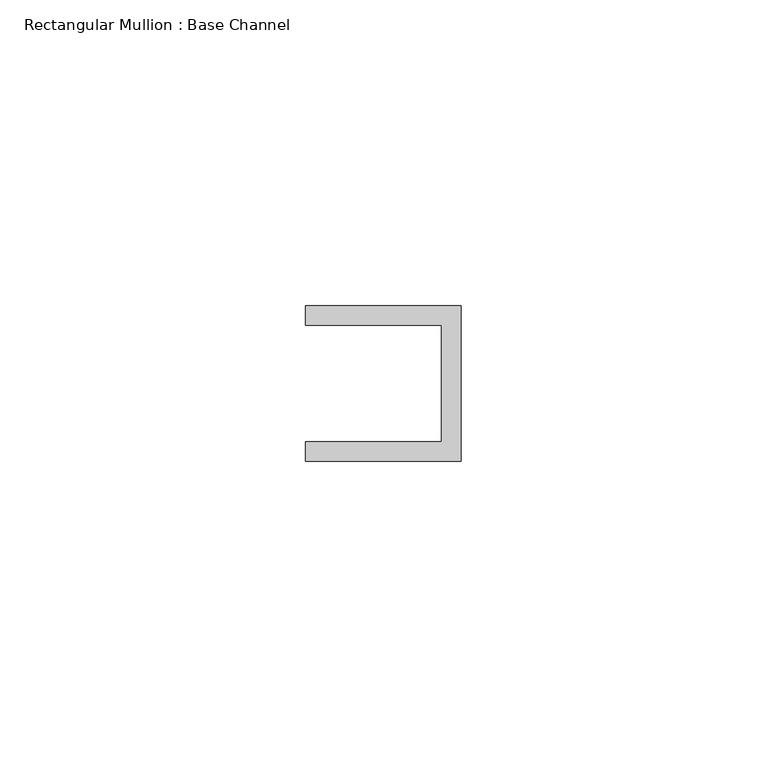
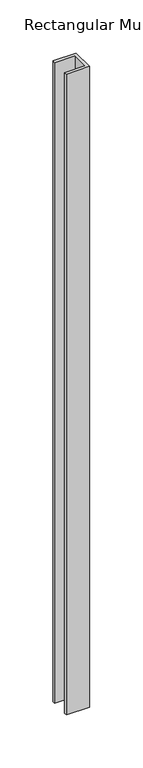
"""IFC4 building model written with IfcOpenShell, lengths in millimetres: member geometry, Rectangular Mullion : Base Channel."""

import ifcopenshell
import ifcopenshell.guid

model = None  # the IFC model being written
_history = None  # IfcOwnerHistory: only IFC2X3 demands one
_inside = {}  # id of a spatial element -> (the spatial element, [elements in it])
_under = {}  # id of a project, library or spatial element -> (it, [spatial elements below it])
_declared = {}  # id of a project -> (the project, [libraries it declares])
_typed = {}  # id of a type object -> (the type object, [elements of that type])
_made_of = {}  # id of a material, layer set ... -> (it, [elements and type objects made of it])


def new_model(schema):
    """Start an empty IFC model of exactly this schema.

    Asked for "IFC4X3", IfcOpenShell would pick the latest addendum, in which some entities
    have other attributes; the version numbers below select the first issue.
    IFC2X3 requires an IfcOwnerHistory on every rooted entity: one is made here for all.
    """
    global model, _history
    if schema == "IFC4X3":
        model = ifcopenshell.file(schema_version=(4, 3, 0, 0))
    else:
        model = ifcopenshell.file(schema=schema)
    _inside.clear()
    _under.clear()
    _declared.clear()
    _typed.clear()
    _made_of.clear()
    _history = None
    if model.schema == "IFC2X3":
        org = make("IfcOrganization", Name="unknown")
        user = make(
            "IfcPersonAndOrganization",
            ThePerson=make("IfcPerson", FamilyName="unknown"),
            TheOrganization=org,
        )
        app = make(
            "IfcApplication",
            ApplicationDeveloper=org,
            Version="unknown",
            ApplicationFullName="unknown",
            ApplicationIdentifier="unknown",
        )
        _history = make(
            "IfcOwnerHistory",
            OwningUser=user,
            OwningApplication=app,
            ChangeAction="ADDED",
            CreationDate=0,
        )
    return model


def make(cls, **values):
    """One entity of the class cls with the attributes given. An attribute that is None is left unset."""
    return model.create_entity(
        cls, **{name: value for name, value in values.items() if value is not None}
    )


def rooted(cls, **values):
    """An entity with a GlobalId (a new one), such as an element, a storey or a relation."""
    return make(cls, GlobalId=ifcopenshell.guid.new(), OwnerHistory=_history, **values)


def si_unit(unit_type, name, prefix=None):
    """IfcSIUnit, for example si_unit("LENGTHUNIT", "METRE", prefix="MILLI")."""
    return make("IfcSIUnit", UnitType=unit_type, Prefix=prefix, Name=name)


def assignment(units):
    """IfcUnitAssignment: the units of a project."""
    return None if units is None else make("IfcUnitAssignment", Units=units)


def point(xyz):
    """IfcCartesianPoint."""
    return None if xyz is None else make("IfcCartesianPoint", Coordinates=xyz)


def direction(xyz):
    """IfcDirection."""
    return None if xyz is None else make("IfcDirection", DirectionRatios=xyz)


def frame(location, z_axis=None, x_axis=None):
    """IfcAxis2Placement3D, a coordinate frame: its origin and axes. An axis left out is left unset."""
    return make(
        "IfcAxis2Placement3D",
        Location=point(location),
        Axis=direction(z_axis),
        RefDirection=direction(x_axis),
    )


def origin():
    """The frame at (0, 0, 0) with its axes left unset."""
    return frame((0.0, 0.0, 0.0))


def place(relative_to, where):
    """IfcLocalPlacement: puts the frame where relative to a parent placement (None: the world)."""
    return make(
        "IfcLocalPlacement", PlacementRelTo=relative_to, RelativePlacement=where
    )


def context(
    kind, dimensions, precision=None, world=None, true_north=None, identifier=None
):
    """IfcGeometricRepresentationContext, for example the 3D "Model" context."""
    return make(
        "IfcGeometricRepresentationContext",
        ContextIdentifier=identifier,
        ContextType=kind,
        CoordinateSpaceDimension=dimensions,
        Precision=precision,
        WorldCoordinateSystem=world,
        TrueNorth=true_north,
    )


def project(units=None, contexts=None):
    """IfcProject with its units and contexts."""
    return rooted(
        "IfcProject",
        Name="project",
        RepresentationContexts=contexts,
        UnitsInContext=assignment(units),
    )


def spatial(cls, under=None, at=None, **own):
    """A site, building, storey or space (cls), placed at a placement, below another one or the project."""
    s = rooted(cls, ObjectPlacement=at, **own)
    if under is not None:
        _under.setdefault(under.id(), (under, []))[1].append(s)
    return s


def polyline(points):
    """IfcPolyline through the points."""
    return make("IfcPolyline", Points=[point(p) for p in points])


def outline(outer, holes=None, kind="AREA"):
    """IfcArbitraryClosedProfileDef: a profile drawn as a closed curve; with holes, ...WithVoids."""
    if holes is None:
        return make("IfcArbitraryClosedProfileDef", ProfileType=kind, OuterCurve=outer)
    return make(
        "IfcArbitraryProfileDefWithVoids",
        ProfileType=kind,
        OuterCurve=outer,
        InnerCurves=holes,
    )


def extrude(swept, where, along, depth):
    """IfcExtrudedAreaSolid: the profile swept, set in the frame where, extruded along a direction by depth."""
    return make(
        "IfcExtrudedAreaSolid",
        SweptArea=swept,
        Position=where,
        ExtrudedDirection=direction(along),
        Depth=depth,
    )


def shape(context_of_items, identifier, shape_type, items):
    """IfcShapeRepresentation: the items that make up one representation, for example the "Body"."""
    return make(
        "IfcShapeRepresentation",
        ContextOfItems=context_of_items,
        RepresentationIdentifier=identifier,
        RepresentationType=shape_type,
        Items=items,
    )


def source(mapping_origin, context_of_items, identifier, shape_type, items):
    """IfcRepresentationMap: a shape defined once, which mapped items show again and again."""
    return make(
        "IfcRepresentationMap",
        MappingOrigin=mapping_origin,
        MappedRepresentation=shape(context_of_items, identifier, shape_type, items),
    )


def transform(
    local_origin,
    x_axis=None,
    y_axis=None,
    z_axis=None,
    scale=None,
    scale2=None,
    scale3=None,
    uniform=True,
):
    """IfcCartesianTransformationOperator3D, or its non-uniform kind. x_axis, y_axis, z_axis: its Axis1, 2, 3."""
    if uniform:
        return make(
            "IfcCartesianTransformationOperator3D",
            Axis1=direction(x_axis),
            Axis2=direction(y_axis),
            LocalOrigin=point(local_origin),
            Scale=scale,
            Axis3=direction(z_axis),
        )
    return make(
        "IfcCartesianTransformationOperator3DnonUniform",
        Axis1=direction(x_axis),
        Axis2=direction(y_axis),
        LocalOrigin=point(local_origin),
        Scale=scale,
        Axis3=direction(z_axis),
        Scale2=scale2,
        Scale3=scale3,
    )


def mapped(mapping_source, mapping_target):
    """IfcMappedItem: shows the shape of a source again, moved by a transform."""
    return make(
        "IfcMappedItem", MappingSource=mapping_source, MappingTarget=mapping_target
    )


def made_of(thing, what):
    """Note that an element or type object is made of a material, layer set ...; save() writes the relation."""
    if what is not None:
        _made_of.setdefault(what.id(), (what, []))[1].append(thing)
    return thing


def element(
    cls,
    number,
    at=None,
    inside=None,
    cuts=None,
    type_object=None,
    material=None,
    context=None,
    identifier="Body",
    shape_type=None,
    held_by="IfcProductDefinitionShape",
    body=None,
    shapes=None,
    **own,
):
    """One element of the class cls, such as IfcWall. Its Tag is "e" and its number.

    at: its placement. inside: the storey or other place that contains it. cuts: it is an
    opening in that element (IfcRelVoidsElement). A single representation is given by context,
    identifier, shape_type and body (its items); several are given by shapes. held_by: the class
    of the entity that holds the representations. save() writes the other relations.
    """
    e = rooted(cls, Tag="e%d" % number, ObjectPlacement=at, **own)
    if body is not None:
        shapes = [shape(context, identifier, shape_type, body)]
    if shapes is not None:
        e.Representation = make(held_by, Representations=shapes)
    if inside is not None:
        _inside.setdefault(inside.id(), (inside, []))[1].append(e)
    if cuts is not None:
        rooted(
            "IfcRelVoidsElement", RelatingBuildingElement=cuts, RelatedOpeningElement=e
        )
    if type_object is not None:
        _typed.setdefault(type_object.id(), (type_object, []))[1].append(e)
    return made_of(e, material)


def aggregate(whole, parts):
    """IfcRelAggregates: a whole, such as a stair, and the parts it consists of."""
    return rooted("IfcRelAggregates", RelatingObject=whole, RelatedObjects=parts)


def save(model, path):
    """Write the relations noted so far, then the file.

    IfcRelAggregates (storeys below a building ...), IfcRelContainedInSpatialStructure (elements
    in a storey), IfcRelDefinesByType, IfcRelAssociatesMaterial and IfcRelDeclares: one each for
    every whole, place, type object, material and project.
    """
    for whole, parts in _under.values():
        aggregate(whole, parts)
    for where, things in _inside.values():
        rooted(
            "IfcRelContainedInSpatialStructure",
            RelatedElements=things,
            RelatingStructure=where,
        )
    for kind, things in _typed.values():
        rooted("IfcRelDefinesByType", RelatedObjects=things, RelatingType=kind)
    for what, things in _made_of.values():
        rooted("IfcRelAssociatesMaterial", RelatedObjects=things, RelatingMaterial=what)
    for by, libraries in _declared.values():
        rooted("IfcRelDeclares", RelatingContext=by, RelatedDefinitions=libraries)
    model.write(path)


def rectangular_mullion_base_channel_0abb9bad(model_context):
    return source(origin(), model_context, "Body", "SweptSolid", [
        extrude(outline(polyline([(0.0, -12.7), (-25.4, -12.7), (-25.4, -9.525), (-3.175, -9.525), (-3.175, 9.525), (-25.4, 9.525), (-25.4, 12.7), (0.0, 12.7), (0.0, -12.7)])), frame((0.0, 0.0, -736.6), z_axis=(0.0, 0.0, 1.0), x_axis=(1.0, 0.0, 0.0)), (0.0, 0.0, 1.0), 736.6),
    ])


if __name__ == "__main__":
    model = new_model("IFC4")
    model_context = context("Model", 3, world=origin())
    ifc_project = project(units=[si_unit("LENGTHUNIT", "METRE", prefix="MILLI")], contexts=[model_context])
    site = spatial("IfcSite", under=ifc_project)
    building = spatial("IfcBuilding", under=site)
    placement = place(None, origin())
    rectangular_mullion_base_channel_shape = rectangular_mullion_base_channel_0abb9bad(model_context)
    element("IfcMember", 1, ObjectType="Rectangular Mullion : Base Channel", at=placement, inside=building, context=model_context, shape_type="MappedRepresentation", body=[
        mapped(rectangular_mullion_base_channel_shape, transform((0.0, 0.0, 0.0), x_axis=(1.0, 0.0, 0.0), y_axis=(0.0, 1.0, 0.0), z_axis=(0.0, 0.0, 1.0))),
    ])
    save(model, "model.ifc")

# Revit data of these elements
# Type "Rectangular Mullion : Base Channel"
#   built-in parameter 1007322 = 0.0833333 (stored number, unit not read)
#   built-in parameter 1007321 = 0.0416667 (stored number, unit not read)
#   built-in parameter 1007320 = -0.03125 (stored number, unit not read)
# Element 1 (IfcMember, "Rectangular Mullion : Base Channel")
#   Materials on its faces: "ALUM"
# Materials
#   "ALUM": class "Generic", colour RGB 157 157 157, transparency 0, Cost = 0
